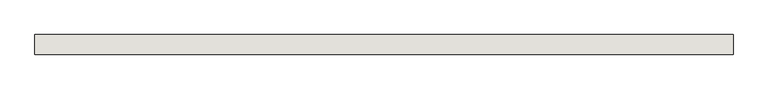
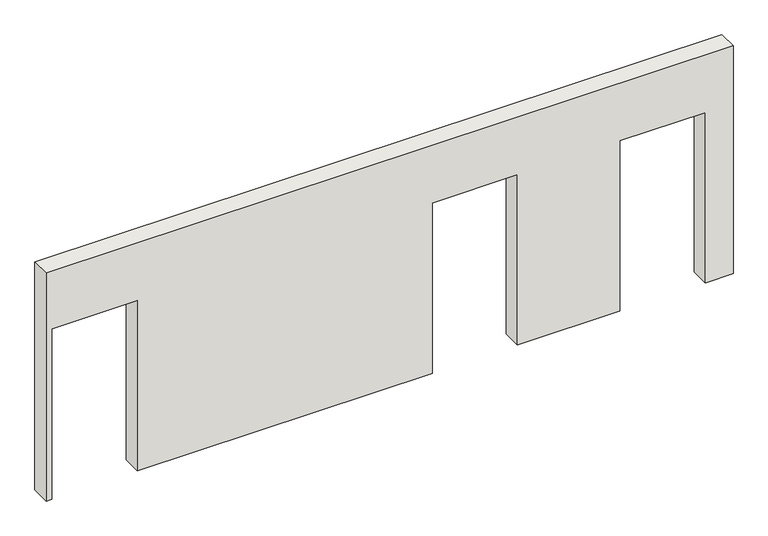
"""IFC4 building model written with IfcOpenShell, lengths in millimetres: wall geometry, Holzwand."""

from ifc_helpers import new_model, si_unit, frame, origin, place, context, project, spatial, polyline, outline, extrude, source, transform, mapped, element, save


def wall_67aac6ca(model_context):
    return source(origin(), model_context, "Body", "SweptSolid", [
        extrude(outline(polyline([(1870.0, 6837.13465), (0.0, 6837.13465), (0.0, 7125.0), (2500.0, 7125.0), (2500.0, 0.0), (0.0, 0.0), (0.0, 60.0), (1870.0, 60.0), (1870.0, 945.0), (0.0, 945.0), (0.0, 4003.8914512), (1870.0, 4003.8914512), (1870.0, 4888.8914512), (0.0, 4888.8914512), (0.0, 5952.13465), (1870.0, 5952.13465), (1870.0, 6837.13465)])), frame((0.0, 0.0, 0.0), z_axis=(0.0, 1.0, 0.0), x_axis=(0.0, 0.0, 1.0)), (0.0, 0.0, 1.0), 200.0),
    ])


if __name__ == "__main__":
    model = new_model("IFC4")
    model_context = context("Model", 3, world=origin())
    ifc_project = project(units=[si_unit("LENGTHUNIT", "METRE", prefix="MILLI")], contexts=[model_context])
    site = spatial("IfcSite", under=ifc_project)
    building = spatial("IfcBuilding", under=site)
    placement = place(None, origin())
    wall_shape = wall_67aac6ca(model_context)
    element("IfcWall", 1, ObjectType="Holzwand", at=placement, inside=building, context=model_context, shape_type="MappedRepresentation", body=[
        mapped(wall_shape, transform((0.0, 0.0, 0.0), x_axis=(1.0, 0.0, 0.0), y_axis=(0.0, 1.0, 0.0), z_axis=(0.0, 0.0, 1.0))),
    ])
    save(model, "model.ifc")

# Revit data of these elements
# Element 1 (IfcWall, "Holzwand")
#   Materials on its faces: "holzschalung"
# Materials
#   "holzschalung": class "Unassigned", colour RGB 128 128 128, transparency 0
